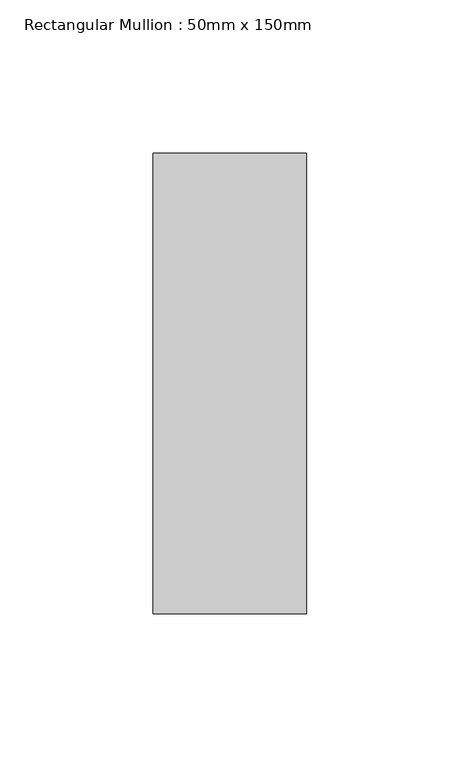
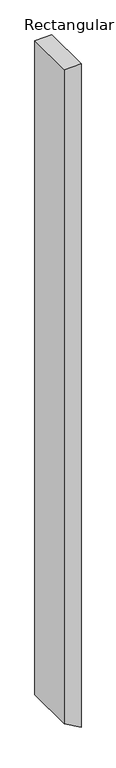
"""IFC4 building model written with IfcOpenShell, lengths in millimetres: member geometry, Rectangular Mullion : 50mm x 150mm."""

from ifc_helpers import new_model, si_unit, frame, origin, place, context, project, spatial, polyline, outline, extrude, source, transform, mapped, element, save


def rectangular_mullion_50mm_x_150mm_5913aded(model_context):
    return source(origin(), model_context, "Body", "SweptSolid", [
        extrude(outline(polyline([(0.0, 25.0), (0.0, -25.0), (-2047.5740063, -25.0), (-2076.4415198, 25.0), (0.0, 25.0)])), frame((0.0, -75.0, 0.0), z_axis=(0.0, 1.0, 0.0), x_axis=(0.0, 0.0, 1.0)), (0.0, 0.0, 1.0), 150.0),
    ])


if __name__ == "__main__":
    model = new_model("IFC4")
    model_context = context("Model", 3, world=origin())
    ifc_project = project(units=[si_unit("LENGTHUNIT", "METRE", prefix="MILLI")], contexts=[model_context])
    site = spatial("IfcSite", under=ifc_project)
    building = spatial("IfcBuilding", under=site)
    placement = place(None, origin())
    rectangular_mullion_50mm_x_150mm_shape = rectangular_mullion_50mm_x_150mm_5913aded(model_context)
    element("IfcMember", 1, ObjectType="Rectangular Mullion : 50mm x 150mm", at=placement, inside=building, context=model_context, shape_type="MappedRepresentation", body=[
        mapped(rectangular_mullion_50mm_x_150mm_shape, transform((0.0, 0.0, 0.0), x_axis=(1.0, 0.0, 0.0), y_axis=(0.0, 1.0, 0.0), z_axis=(0.0, 0.0, 1.0))),
    ])
    save(model, "model.ifc")

# Revit data of these elements
# Type "Rectangular Mullion : 50mm x 150mm"
#   built-in parameter 1007304 = 0.492126 (stored number, unit not read)
#   built-in parameter 1007301 = 0.082021 (stored number, unit not read)
#   built-in parameter 1007300 = 0.082021 (stored number, unit not read)
# Element 1 (IfcMember, "Rectangular Mullion : 50mm x 150mm")
#   Materials on its faces: "Aluminum"
# Materials
#   "Aluminum": class "Metal", colour RGB 247 247 247, transparency 0, Description = "Aluminum 6061", Cost = 0
